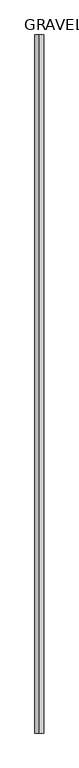
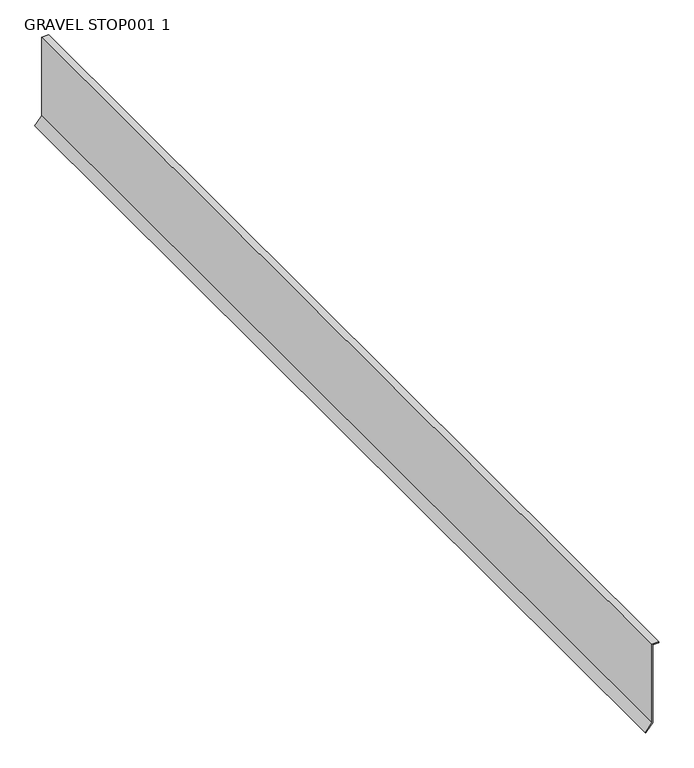
"""IFC4 building model written with IfcOpenShell, lengths in millimetres: proxy geometry, GRAVEL STOP001 1 : GRAVEL STOP001 15288."""

from ifc_helpers import new_model, si_unit, frame, origin, place, context, project, spatial, polyline, outline, extrude, source, transform, mapped, element, save


def gravel_stop001_1_e2b98164(model_context):
    return source(origin(), model_context, "Body", "SweptSolid", [
        extrude(outline(polyline([(40082.2407116, -2815.6343429), (40081.3605882, -2814.5313394), (40097.4918556, -2801.659661), (40253.3245993, -2801.659661), (40253.3245993, -2789.8917422), (40254.7357103, -2789.8917422), (40254.7357103, -2803.070772), (40097.9858473, -2803.070772), (40082.2407116, -2815.6343429)])), frame((0.0, -1052.8906573, 0.0), z_axis=(0.0, 1.0, 0.0), x_axis=(0.0, 0.0, 1.0)), (0.0, 0.0, 1.0), 2000.25),
    ])


if __name__ == "__main__":
    model = new_model("IFC4")
    model_context = context("Model", 3, world=origin())
    ifc_project = project(units=[si_unit("LENGTHUNIT", "METRE", prefix="MILLI")], contexts=[model_context])
    site = spatial("IfcSite", under=ifc_project)
    building = spatial("IfcBuilding", under=site)
    placement = place(None, origin())
    gravel_stop001_1_shape = gravel_stop001_1_e2b98164(model_context)
    element("IfcBuildingElementProxy", 1, Name="GRAVEL STOP001 1 : GRAVEL STOP001 15288", ObjectType="GRAVEL STOP001 1 : GRAVEL STOP001 15288", at=placement, inside=building, context=model_context, shape_type="MappedRepresentation", body=[
        mapped(gravel_stop001_1_shape, transform((0.0, 0.0, 0.0), x_axis=(1.0, 0.0, 0.0), y_axis=(0.0, 1.0, 0.0), z_axis=(0.0, 0.0, 1.0))),
    ])
    save(model, "model.ifc")

# Revit data of these elements
# Type "GRAVEL STOP001 1 : GRAVEL STOP001 15288"
#   NameOverride = "GRAVEL STOP001"
# Element 1 (IfcBuildingElementProxy, "GRAVEL STOP001 1 : GRAVEL STOP001 15288")
#   Materials on its faces: "GRAVEL STOP REQUIRED WITH GRAVEL SURFACE SYSTEMS"
# Materials
#   "GRAVEL STOP REQUIRED WITH GRAVEL SURFACE SYSTEMS": class "Unassigned", colour RGB 170 170 127, transparency 0, Cost = 0
